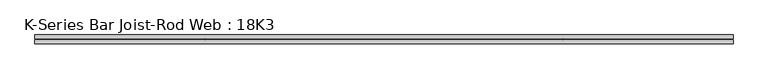
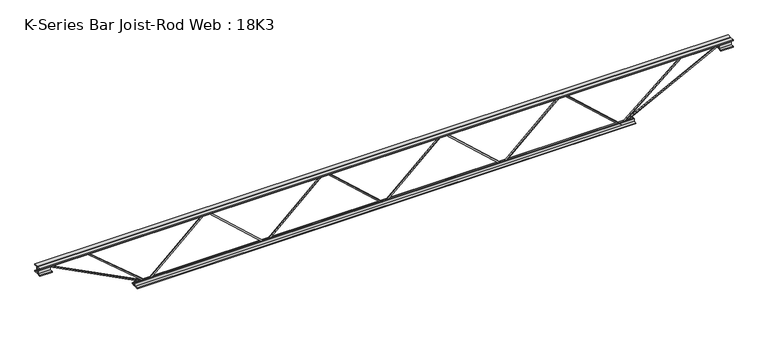
"""IFC4 building model written with IfcOpenShell, lengths in millimetres: beam geometry, K-Series Bar Joist-Rod Web : 18K3."""

from ifc_helpers import new_model, si_unit, frame, origin, place, context, project, spatial, polyline, outline, extrude, source, transform, mapped, element, save


def k_series_bar_joist_rod_web_18k3_71307e8f(model_context):
    return source(origin(), model_context, "Body", "SweptSolid", [
        extrude(outline(polyline([(-217.4875, 0.0), (-227.0125, 0.0), (-227.0125, 5.0162152), (217.4875, 493.9662152), (217.4875, 496.6337848), (-227.0125, 985.5837848), (-227.0125, 990.6), (-217.4875, 990.6), (-217.4875, 989.2662152), (227.0125, 500.3162152), (227.0125, 490.2837848), (-217.4875, 1.3337848), (-217.4875, 0.0)])), frame((0.0, -4.7625, 0.0), z_axis=(0.0, 1.0, 0.0), x_axis=(0.0, 0.0, 1.0)), (0.0, 0.0, 1.0), 9.525),
        extrude(outline(polyline([(-217.4875, -990.6), (-227.0125, -990.6), (-227.0125, -985.5837848), (217.4875, -496.6337848), (217.4875, -493.9662152), (-227.0125, -5.0162152), (-227.0125, 0.0), (-217.4875, 0.0), (-217.4875, -1.3337848), (227.0125, -490.2837848), (227.0125, -500.3162152), (-217.4875, -989.2662152), (-217.4875, -990.6)])), frame((0.0, -4.7625, 0.0), z_axis=(0.0, 1.0, 0.0), x_axis=(0.0, 0.0, 1.0)), (0.0, 0.0, 1.0), 9.525),
        extrude(outline(polyline([(-217.4875, 990.6), (-227.0125, 990.6), (-227.0125, 995.6162152), (217.4875, 1484.5662152), (217.4875, 1487.2337848), (-227.0125, 1976.1837848), (-227.0125, 1981.2), (-217.4875, 1981.2), (-217.4875, 1979.8662152), (227.0125, 1490.9162152), (227.0125, 1480.8837848), (-217.4875, 991.9337848), (-217.4875, 990.6)])), frame((0.0, -4.7625, 0.0), z_axis=(0.0, 1.0, 0.0), x_axis=(0.0, 0.0, 1.0)), (0.0, 0.0, 1.0), 9.525),
        extrude(outline(polyline([(-217.4875, -1981.2), (-227.0125, -1981.2), (-227.0125, -1976.1837848), (217.4875, -1487.2337848), (217.4875, -1484.5662152), (-227.0125, -995.6162152), (-227.0125, -990.6), (-217.4875, -990.6), (-217.4875, -991.9337848), (227.0125, -1480.8837848), (227.0125, -1490.9162152), (-217.4875, -1979.8662152), (-217.4875, -1981.2)])), frame((0.0, -4.7625, 0.0), z_axis=(0.0, 1.0, 0.0), x_axis=(0.0, 0.0, 1.0)), (0.0, 0.0, 1.0), 9.525),
        extrude(outline(polyline([(4.7625, 228.6), (36.5125, 228.6), (36.5125, 222.25), (11.1125, 222.25), (11.1125, 196.85), (4.7625, 196.85), (4.7625, 228.6)])), frame((-2895.6, 0.0, 0.0), z_axis=(1.0, 0.0, 0.0), x_axis=(0.0, 1.0, 0.0)), (0.0, 0.0, 1.0), 5791.2),
        extrude(outline(polyline([(-4.7625, 228.6), (-4.7625, 196.85), (-11.1125, 196.85), (-11.1125, 222.25), (-36.5125, 222.25), (-36.5125, 228.6), (-4.7625, 228.6)])), frame((-2895.6, 0.0, 0.0), z_axis=(1.0, 0.0, 0.0), x_axis=(0.0, 1.0, 0.0)), (0.0, 0.0, 1.0), 5791.2),
        extrude(outline(polyline([(-4.7625, 165.1), (-36.5125, 165.1), (-36.5125, 171.45), (-11.1125, 171.45), (-11.1125, 196.85), (-4.7625, 196.85), (-4.7625, 165.1)])), frame((-2895.6, 0.0, 0.0), z_axis=(1.0, 0.0, 0.0), x_axis=(0.0, 1.0, 0.0)), (0.0, 0.0, 1.0), 101.6),
        extrude(outline(polyline([(36.5125, 165.1), (4.7625, 165.1), (4.7625, 196.85), (11.1125, 196.85), (11.1125, 171.45), (36.5125, 171.45), (36.5125, 165.1)])), frame((-2895.6, 0.0, 0.0), z_axis=(1.0, 0.0, 0.0), x_axis=(0.0, 1.0, 0.0)), (0.0, 0.0, 1.0), 101.6),
        extrude(outline(polyline([(4.7625, 165.1), (4.7625, 196.85), (11.1125, 196.85), (11.1125, 171.45), (36.5125, 171.45), (36.5125, 165.1), (4.7625, 165.1)])), frame((2794.0, 0.0, 0.0), z_axis=(1.0, 0.0, 0.0), x_axis=(0.0, 1.0, 0.0)), (0.0, 0.0, 1.0), 101.6),
        extrude(outline(polyline([(-4.7625, 165.1), (-36.5125, 165.1), (-36.5125, 171.45), (-11.1125, 171.45), (-11.1125, 196.85), (-4.7625, 196.85), (-4.7625, 165.1)])), frame((2794.0, 0.0, 0.0), z_axis=(1.0, 0.0, 0.0), x_axis=(0.0, 1.0, 0.0)), (0.0, 0.0, 1.0), 101.6),
        extrude(outline(polyline([(4.7625, -228.6), (4.7625, -196.85), (11.1125, -196.85), (11.1125, -222.25), (36.5125, -222.25), (36.5125, -228.6), (4.7625, -228.6)])), frame((-2082.8, 0.0, 0.0), z_axis=(1.0, 0.0, 0.0), x_axis=(0.0, 1.0, 0.0)), (0.0, 0.0, 1.0), 4165.6),
        extrude(outline(polyline([(-4.7625, -228.6), (-36.5125, -228.6), (-36.5125, -222.25), (-11.1125, -222.25), (-11.1125, -196.85), (-4.7625, -196.85), (-4.7625, -228.6)])), frame((-2082.8, 0.0, 0.0), z_axis=(1.0, 0.0, 0.0), x_axis=(0.0, 1.0, 0.0)), (0.0, 0.0, 1.0), 4165.6),
        extrude(outline(polyline([(0.0, -9.525), (0.0, 0.0), (914.4881902, 0.0), (914.4881902, -9.525), (0.0, -9.525)])), frame((-2796.182602, 4.7625, 192.6170749), z_axis=(0.4582891331947272, 0.0, 0.888803167408637), x_axis=(0.888803167408637, 0.0, -0.4582891331947272)), (0.0, 0.0, 1.0), 9.525),
        extrude(outline(polyline([(0.0, -9.525), (0.0, 0.0), (648.8196205, 0.0), (648.8196205, -9.525), (0.0, -9.525)])), frame((-2479.5762999, 4.7625, 193.2143728), z_axis=(0.6459422414659064, 0.0, 0.7633862853693409), x_axis=(0.7633862853693409, 0.0, -0.6459422414659064)), (0.0, 0.0, 1.0), 9.525),
        extrude(outline(polyline([(0.0, -9.525), (0.0, 0.0), (914.4881902, 0.0), (914.4881902, -9.525), (0.0, -9.525)])), frame((2796.182602, -4.7625, 192.6170749), z_axis=(-0.458289133194716, 0.0, 0.8888031674086428), x_axis=(-0.8888031674086428, 0.0, -0.458289133194716)), (0.0, 0.0, 1.0), 9.525),
        extrude(outline(polyline([(0.0, -9.525), (0.0, 0.0), (648.8196205, 0.0), (648.8196205, -9.525), (0.0, -9.525)])), frame((2479.5762999, -4.7625, 193.2143728), z_axis=(-0.6459422414659022, 0.0, 0.7633862853693444), x_axis=(-0.7633862853693444, 0.0, -0.6459422414659022)), (0.0, 0.0, 1.0), 9.525),
    ])


if __name__ == "__main__":
    model = new_model("IFC4")
    model_context = context("Model", 3, world=origin())
    ifc_project = project(units=[si_unit("LENGTHUNIT", "METRE", prefix="MILLI")], contexts=[model_context])
    site = spatial("IfcSite", under=ifc_project)
    building = spatial("IfcBuilding", under=site)
    placement = place(None, origin())
    k_series_bar_joist_rod_web_18k3_shape = k_series_bar_joist_rod_web_18k3_71307e8f(model_context)
    element("IfcBeam", 1, ObjectType="K-Series Bar Joist-Rod Web : 18K3", at=placement, inside=building, context=model_context, shape_type="MappedRepresentation", body=[
        mapped(k_series_bar_joist_rod_web_18k3_shape, transform((0.0, 0.0, 0.0), x_axis=(1.0, 0.0, 0.0), y_axis=(0.0, 1.0, 0.0), z_axis=(0.0, 0.0, 1.0))),
    ])
    save(model, "model.ifc")

# Revit data of these elements
# Type "K-Series Bar Joist-Rod Web : 18K3"
#   Assembly Code = "B1010350"
#   Wt = 6.6
#   Web Thickness = 0' - 0 3/8"
#   Start Offset [instance default] = 0' - 0"
#   Start Extension [instance default] = 0' - 0"
#   Seat Length = 0' - 4"
#   Seat Depth = 0' - 2 1/2"
#   PanelArrayLength [instance default] = 18' - 0"
#   Panel [instance default] = 3' - 0"
#   End Offset [instance default] = 0' - 0"
#   End Extension [instance default] = 0' - 0"
#   End Panel = 3' - 0"
#   Cord Leg = 0' - 1 1/4"
#   Chord Thickness = 0' - 0 1/4"
#   Length [instance default] = 24' - 0"
#   Depth = 1' - 6"
#   PanelArrayNum [instance default] = 6
#   Structural Material = none
# Element 1 (IfcBeam, "K-Series Bar Joist-Rod Web : 18K3")
#   PanelArrayLength = 13' - 0"
#   Panel = 3' - 3"
#   PanelArrayNum = 4
